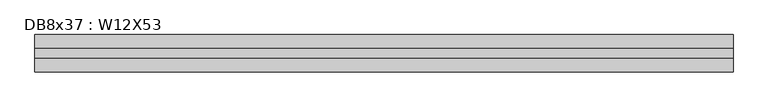
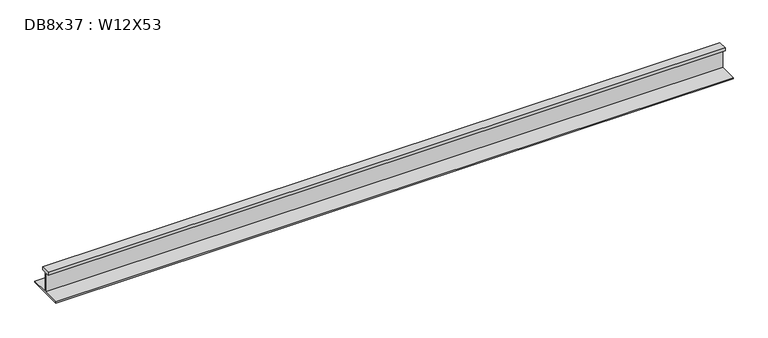
"""IFC4 building model written with IfcOpenShell, lengths in millimetres: beam geometry, DB8x37 : W12X53."""

from ifc_helpers import new_model, si_unit, frame, origin, place, context, project, spatial, polyline, outline, extrude, source, transform, mapped, element, save


def db8x37_w12x53_54ed7fd7(model_context):
    return source(origin(), model_context, "Body", "SweptSolid", [
        extrude(outline(polyline([(38.1, 145.415), (38.1, 120.015), (2.921, 120.015), (2.921, -48.4505), (152.4, -48.4505), (152.4, -58.1025), (-152.4, -58.1025), (-152.4, -48.4505), (-2.921, -48.4505), (-2.921, 120.015), (-38.1, 120.015), (-38.1, 145.415), (38.1, 145.415)])), frame((-2832.0999994, 0.0, 0.0), z_axis=(1.0, 0.0, 0.0), x_axis=(0.0, 1.0, 0.0)), (0.0, 0.0, 1.0), 5664.1999988),
    ])


if __name__ == "__main__":
    model = new_model("IFC4")
    model_context = context("Model", 3, world=origin())
    ifc_project = project(units=[si_unit("LENGTHUNIT", "METRE", prefix="MILLI")], contexts=[model_context])
    site = spatial("IfcSite", under=ifc_project)
    building = spatial("IfcBuilding", under=site)
    placement = place(None, origin())
    db8x37_w12x53_shape = db8x37_w12x53_54ed7fd7(model_context)
    element("IfcBeam", 1, ObjectType="DB8x37 : W12X53", at=placement, inside=building, context=model_context, shape_type="MappedRepresentation", body=[
        mapped(db8x37_w12x53_shape, transform((0.0, 0.0, 0.0), x_axis=(1.0, 0.0, 0.0), y_axis=(0.0, 1.0, 0.0), z_axis=(0.0, 0.0, 1.0))),
    ])
    save(model, "model.ifc")

# Revit data of these elements
# Type "DB8x37 : W12X53"
#   Assembly Code = "B10"
#   W = 53
#   Length [instance default] = 5' - 0"
#   bf = 0' - 10"
#   d = 1' - 0.1"
#   k = 0' - 1 3/8"
#   k2 = 0' - 0.8"
#   tf = 0' - 0.575"
#   tw = 0' - 0.345"
#   A = 0.108333 SF
#   Structural Material [instance default] = Steel ASTM A992
# Element 1 (IfcBeam, "DB8x37 : W12X53")
#   Materials on its faces: "Steel ASTM A992"
# Materials
#   "Steel ASTM A992": class "Metal", colour RGB 199 199 199, transparency 0, Description = "Structural steel 50ksi", Cost = 0
